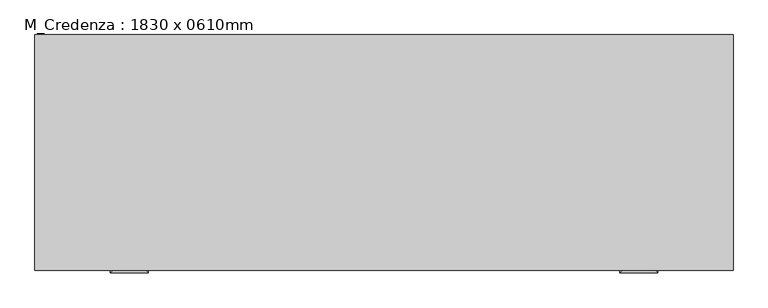
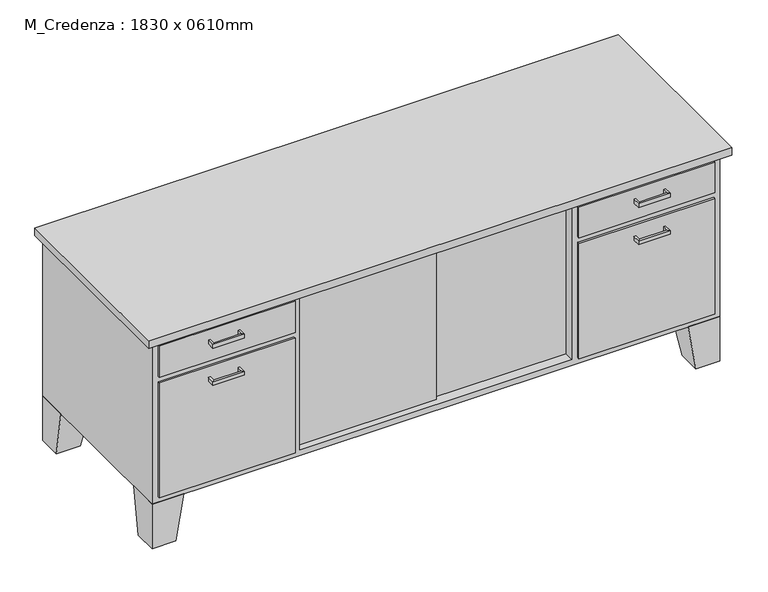
"""IFC4 building model written with IfcOpenShell, lengths in millimetres: furniture geometry, M_Credenza : 1830 x 0610mm."""

from ifc_helpers import new_model, si_unit, frame, origin, place, context, project, spatial, polyline, outline, extrude, faceted_brep, source, transform, mapped, element, save


def m_credenza_1830_x_0610mm_1080a9db(model_context):
    return source(origin(), model_context, "Body", "SolidModel", [
        extrude(outline(polyline([(532.0023176, -267.0714583), (46.8442623, -267.0714583), (46.8442623, -254.7714583), (532.0023176, -254.7714583), (532.0023176, -267.0714583)])), frame((0.0, 0.0, 171.45), z_axis=(0.0, 0.0, 1.0), x_axis=(1.0, 0.0, 0.0)), (0.0, 0.0, 1.0), 518.1),
        extrude(outline(polyline([(73.6254475, -279.7714583), (-378.9057377, -279.7714583), (-378.9057377, -267.0714583), (73.6254475, -267.0714583), (73.6254475, -279.7714583)])), frame((0.0, 0.0, 171.45), z_axis=(0.0, 0.0, 1.0), x_axis=(1.0, 0.0, 0.0)), (0.0, 0.0, 1.0), 518.1),
        faceted_brep([(872.9442623, 309.5803279, 152.4), (872.9442623, 207.9803279, 152.4), (974.5442623, 207.9803279, 152.4), (974.5442623, 309.5803279, 152.4), (898.3442623, 309.5803279, 0.0), (974.5442623, 309.5803279, 0.0), (974.5442623, 233.3803279, 0.0), (898.3442623, 233.3803279, 0.0)], [[[0, 1, 2, 3]], [[4, 5, 6, 7]], [[4, 7, 1, 0]], [[7, 6, 2, 1]], [[6, 5, 3, 2]], [[5, 4, 0, 3]]]),
        extrude(outline(polyline([(955.4942623, -306.3696721), (517.0442623, -306.3696721), (517.0442623, -300.0196721), (955.4942623, -300.0196721), (955.4942623, -306.3696721)])), frame((0.0, 0.0, 584.2), z_axis=(0.0, 0.0, 1.0), x_axis=(1.0, 0.0, 0.0)), (0.0, 0.0, 1.0), 105.35),
        extrude(outline(polyline([(955.4942623, -306.3696721), (517.0442623, -306.3696721), (517.0442623, -300.0196721), (955.4942623, -300.0196721), (955.4942623, -306.3696721)])), frame((0.0, 0.0, 171.45), z_axis=(0.0, 0.0, 1.0), x_axis=(1.0, 0.0, 0.0)), (0.0, 0.0, 1.0), 393.7),
        extrude(outline(polyline([(-397.9557377, -306.7696721), (-836.4057377, -306.7696721), (-836.4057377, -300.4196721), (-397.9557377, -300.4196721), (-397.9557377, -306.7696721)])), frame((0.0, 0.0, 581.6), z_axis=(0.0, 0.0, 1.0), x_axis=(1.0, 0.0, 0.0)), (0.0, 0.0, 1.0), 107.95),
        extrude(outline(polyline([(-397.9557377, -306.7696721), (-836.4057377, -306.7696721), (-836.4057377, -300.4196721), (-397.9557377, -300.4196721), (-397.9557377, -306.7696721)])), frame((0.0, 0.0, 171.45), z_axis=(0.0, 0.0, 1.0), x_axis=(1.0, 0.0, 0.0)), (0.0, 0.0, 1.0), 391.1),
        faceted_brep([(-753.8557377, -300.4196721, 152.4), (-753.8557377, -198.8196721, 152.4), (-855.4557377, -198.8196721, 152.4), (-855.4557377, -300.4196721, 152.4), (-779.2557377, -300.4196721, 0.0), (-855.4557377, -300.4196721, 0.0), (-855.4557377, -224.2196721, 0.0), (-779.2557377, -224.2196721, 0.0)], [[[0, 1, 2, 3]], [[4, 5, 6, 7]], [[4, 7, 1, 0]], [[7, 6, 2, 1]], [[6, 5, 3, 2]], [[5, 4, 0, 3]]]),
        faceted_brep([(-753.8557377, 309.5803279, 152.4), (-855.4557377, 309.5803279, 152.4), (-855.4557377, 207.9803279, 152.4), (-753.8557377, 207.9803279, 152.4), (-779.2557377, 309.5803279, 0.0), (-779.2557377, 233.3803279, 0.0), (-855.4557377, 233.3803279, 0.0), (-855.4557377, 309.5803279, 0.0)], [[[0, 1, 2, 3]], [[4, 5, 6, 7]], [[4, 7, 1, 0]], [[7, 6, 2, 1]], [[6, 5, 3, 2]], [[5, 4, 0, 3]]]),
        faceted_brep([(872.9442623, -300.4196721, 152.4), (974.5442623, -300.4196721, 152.4), (974.5442623, -198.8196721, 152.4), (872.9442623, -198.8196721, 152.4), (898.3442623, -300.4196721, 0.0), (898.3442623, -224.2196721, 0.0), (974.5442623, -224.2196721, 0.0), (974.5442623, -300.4196721, 0.0)], [[[0, 1, 2, 3]], [[4, 5, 6, 7]], [[4, 7, 1, 0]], [[7, 6, 2, 1]], [[6, 5, 3, 2]], [[5, 4, 0, 3]]]),
        faceted_brep([(974.5442623, 309.5803279, 708.6), (-855.4557377, 309.5803279, 708.6), (-855.4557377, -300.4196721, 708.6), (974.5442623, -300.4196721, 708.6), (974.5442623, 309.5803279, 152.4), (974.5442623, -300.4196721, 152.4), (-855.4557377, -300.4196721, 152.4), (-855.4557377, 309.5803279, 152.4), (-378.9057377, -300.4196721, 689.55), (497.9942623, -300.4196721, 689.55), (497.9942623, -300.4196721, 171.45), (-378.9057377, -300.4196721, 171.45), (497.9942623, 290.3303279, 689.55), (-378.9057377, 290.3303279, 689.55), (-378.9057377, 290.3303279, 171.45), (497.9942623, 290.3303279, 171.45)], [[[0, 1, 2, 3]], [[4, 5, 6, 7]], [[1, 0, 4, 7]], [[2, 1, 7, 6]], [[3, 2, 6, 5], [8, 9, 10, 11]], [[0, 3, 5, 4]], [[12, 13, 14, 15]], [[13, 12, 9, 8]], [[14, 13, 8, 11]], [[15, 14, 11, 10]], [[12, 15, 10, 9]]]),
        extrude(outline(polyline([(999.9442623, 309.5803279), (999.9442623, -325.8196721), (-880.8557377, -325.8196721), (-880.8557377, 309.5803279), (999.9442623, 309.5803279)])), frame((0.0, 0.0, 708.6), z_axis=(0.0, 0.0, 1.0), x_axis=(1.0, 0.0, 0.0)), (0.0, 0.0, 1.0), 25.4),
        faceted_brep([(-671.1557377, -306.7696721, 527.05), (-671.1557377, -306.7696721, 514.35), (-677.5057377, -306.7696721, 514.35), (-677.5057377, -306.7696721, 527.05), (-671.1557377, -325.8196721, 527.05), (-671.1557377, -325.8196721, 514.35), (-677.5057377, -332.1696721, 514.35), (-677.5057377, -332.1696721, 527.05), (-582.2557377, -325.8196721, 527.05), (-582.2557377, -325.8196721, 514.35), (-575.9057377, -332.1696721, 514.35), (-575.9057377, -332.1696721, 527.05), (-582.2557377, -306.7696721, 527.05), (-575.9057377, -306.7696721, 527.05), (-575.9057377, -306.7696721, 514.35), (-582.2557377, -306.7696721, 514.35)], [[[0, 1, 2, 3]], [[1, 0, 4, 5]], [[2, 1, 5, 6]], [[3, 2, 6, 7]], [[0, 3, 7, 4]], [[5, 4, 8, 9]], [[6, 5, 9, 10]], [[7, 6, 10, 11]], [[4, 7, 11, 8]], [[12, 13, 14, 15]], [[9, 8, 12, 15]], [[10, 9, 15, 14]], [[11, 10, 14, 13]], [[8, 11, 13, 12]]]),
        faceted_brep([(-671.1557377, -306.7696721, 654.05), (-671.1557377, -306.7696721, 641.35), (-677.5057377, -306.7696721, 641.35), (-677.5057377, -306.7696721, 654.05), (-671.1557377, -325.8196721, 654.05), (-671.1557377, -325.8196721, 641.35), (-677.5057377, -332.1696721, 641.35), (-677.5057377, -332.1696721, 654.05), (-582.2557377, -325.8196721, 654.05), (-582.2557377, -325.8196721, 641.35), (-575.9057377, -332.1696721, 641.35), (-575.9057377, -332.1696721, 654.05), (-582.2557377, -306.7696721, 654.05), (-575.9057377, -306.7696721, 654.05), (-575.9057377, -306.7696721, 641.35), (-582.2557377, -306.7696721, 641.35)], [[[0, 1, 2, 3]], [[1, 0, 4, 5]], [[2, 1, 5, 6]], [[3, 2, 6, 7]], [[0, 3, 7, 4]], [[5, 4, 8, 9]], [[6, 5, 9, 10]], [[7, 6, 10, 11]], [[4, 7, 11, 8]], [[12, 13, 14, 15]], [[9, 8, 12, 15]], [[10, 9, 15, 14]], [[11, 10, 14, 13]], [[8, 11, 13, 12]]]),
        faceted_brep([(701.3442623, -306.7696721, 654.1373112), (701.3442623, -306.7696721, 641.4373112), (694.9942623, -306.7696721, 641.4373112), (694.9942623, -306.7696721, 654.1373112), (701.3442623, -325.8196721, 654.1373112), (701.3442623, -325.8196721, 641.4373112), (694.9942623, -332.1696721, 641.4373112), (694.9942623, -332.1696721, 654.1373112), (790.2442623, -325.8196721, 654.1373112), (790.2442623, -325.8196721, 641.4373112), (796.5942623, -332.1696721, 641.4373112), (796.5942623, -332.1696721, 654.1373112), (790.2442623, -306.7696721, 654.1373112), (796.5942623, -306.7696721, 654.1373112), (796.5942623, -306.7696721, 641.4373112), (790.2442623, -306.7696721, 641.4373112)], [[[0, 1, 2, 3]], [[1, 0, 4, 5]], [[2, 1, 5, 6]], [[3, 2, 6, 7]], [[0, 3, 7, 4]], [[5, 4, 8, 9]], [[6, 5, 9, 10]], [[7, 6, 10, 11]], [[4, 7, 11, 8]], [[12, 13, 14, 15]], [[9, 8, 12, 15]], [[10, 9, 15, 14]], [[11, 10, 14, 13]], [[8, 11, 13, 12]]]),
        faceted_brep([(701.3442623, -306.7696721, 527.05), (701.3442623, -306.7696721, 514.35), (694.9942623, -306.7696721, 514.35), (694.9942623, -306.7696721, 527.05), (701.3442623, -325.8196721, 527.05), (701.3442623, -325.8196721, 514.35), (694.9942623, -332.1696721, 514.35), (694.9942623, -332.1696721, 527.05), (790.2442623, -325.8196721, 527.05), (790.2442623, -325.8196721, 514.35), (796.5942623, -332.1696721, 514.35), (796.5942623, -332.1696721, 527.05), (790.2442623, -306.7696721, 527.05), (796.5942623, -306.7696721, 527.05), (796.5942623, -306.7696721, 514.35), (790.2442623, -306.7696721, 514.35)], [[[0, 1, 2, 3]], [[1, 0, 4, 5]], [[2, 1, 5, 6]], [[3, 2, 6, 7]], [[0, 3, 7, 4]], [[5, 4, 8, 9]], [[6, 5, 9, 10]], [[7, 6, 10, 11]], [[4, 7, 11, 8]], [[12, 13, 14, 15]], [[9, 8, 12, 15]], [[10, 9, 15, 14]], [[11, 10, 14, 13]], [[8, 11, 13, 12]]]),
    ])


if __name__ == "__main__":
    model = new_model("IFC4")
    model_context = context("Model", 3, world=origin())
    ifc_project = project(units=[si_unit("LENGTHUNIT", "METRE", prefix="MILLI")], contexts=[model_context])
    site = spatial("IfcSite", under=ifc_project)
    building = spatial("IfcBuilding", under=site)
    placement = place(None, origin())
    m_credenza_1830_x_0610mm_shape = m_credenza_1830_x_0610mm_1080a9db(model_context)
    element("IfcFurniture", 1, ObjectType="M_Credenza : 1830 x 0610mm", at=placement, inside=building, context=model_context, shape_type="MappedRepresentation", body=[
        mapped(m_credenza_1830_x_0610mm_shape, transform((0.0, 0.0, 0.0), x_axis=(1.0, 0.0, 0.0), y_axis=(0.0, 1.0, 0.0), z_axis=(0.0, 0.0, 1.0))),
    ])
    save(model, "model.ifc")

# Revit data of these elements
# Type "M_Credenza : 1830 x 0610mm"
#   Depth = 0.61 m
#   Height = 0.734 m
#   Width = 1.83 m
#   Desk-Body = Laminate, Ivory, Matte
#   Handle/Leg Material = Steel, Chrome Plated
#   Top Material = Cherry
#   Default Elevation = 0
# Element 1 (IfcFurniture, "M_Credenza : 1830 x 0610mm")
#   Materials on its faces: "Steel, Chrome Plated", "Laminate, Ivory, Matte", "Cherry"
# Materials
#   "Laminate, Ivory, Matte": class "Plastic", colour RGB 247 247 229, transparency 0, Description = "Plastic Laminate - Ivory, Matte", Cost = 0
#   "Steel, Chrome Plated": class "Metal", colour RGB 244 244 244, transparency 0, Description = "Chromiuim plated steel", Cost = 0
#   "Cherry": class "Wood", colour RGB 157 77 38, transparency 0, Description = "Prunus Serotina", Cost = 0
